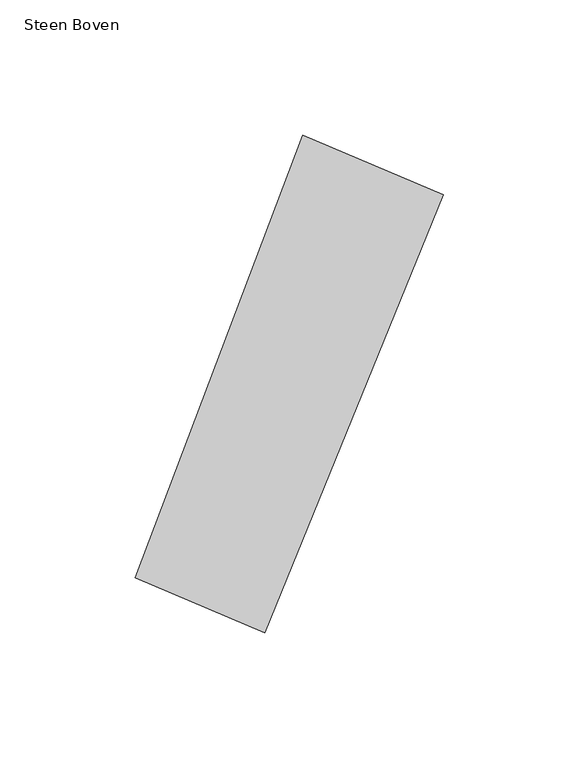
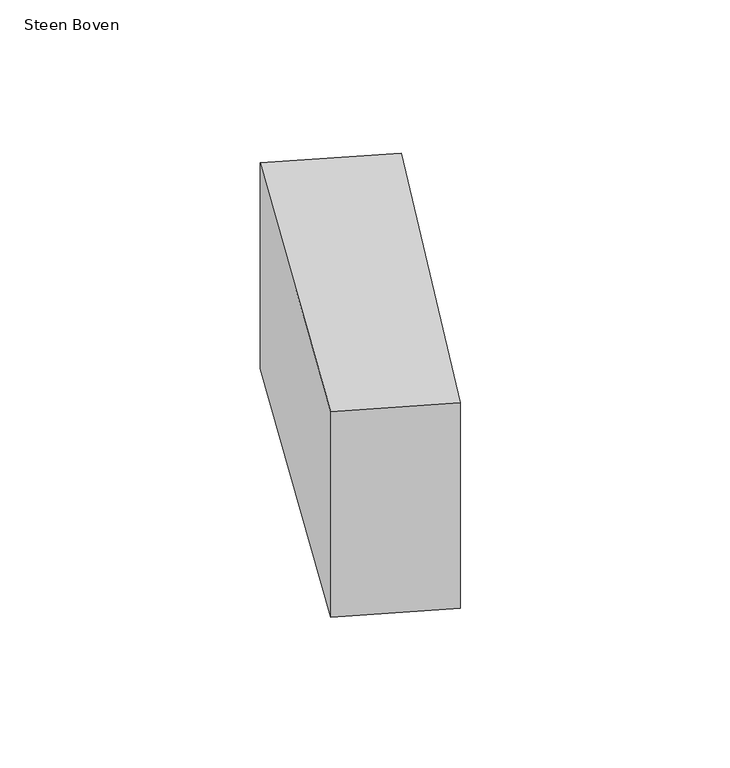
"""IFC4 building model written with IfcOpenShell, lengths in millimetres: proxy geometry, 00_GMA_steen_versie_4 : Steen Boven."""

from ifc_helpers import new_model, si_unit, origin, origin_with_axes, place, context, project, spatial, polyline, outline, extrude, source, transform, mapped, element, save


def steen_boven_43825531(model_context):
    return source(origin(), model_context, "Body", "SweptSolid", [
        extrude(outline(polyline([(135.0092648, 153.8651447), (68.783702, -8.1375562), (20.9158232, 12.1762368), (82.8466643, 176.0050232), (135.0092648, 153.8651447)])), origin_with_axes(), (0.0, 0.0, 1.0), 100.0),
    ])


if __name__ == "__main__":
    model = new_model("IFC4")
    model_context = context("Model", 3, world=origin())
    ifc_project = project(units=[si_unit("LENGTHUNIT", "METRE", prefix="MILLI")], contexts=[model_context])
    site = spatial("IfcSite", under=ifc_project)
    building = spatial("IfcBuilding", under=site)
    placement = place(None, origin())
    steen_boven_shape = steen_boven_43825531(model_context)
    element("IfcBuildingElementProxy", 1, Name="00_GMA_steen_versie_4 : Steen Boven", ObjectType="00_GMA_steen_versie_4 : Steen Boven", at=placement, inside=building, context=model_context, shape_type="MappedRepresentation", body=[
        mapped(steen_boven_shape, transform((0.0, 0.0, 0.0), x_axis=(1.0, 0.0, 0.0), y_axis=(0.0, 1.0, 0.0), z_axis=(0.0, 0.0, 1.0))),
    ])
    save(model, "model.ifc")

# Revit data of these elements
# Type "00_GMA_steen_versie_4 : Steen Boven"
#   StootVoegHalfBoven [instance default] = 5 mm
#   StootVoegHalf [instance default] = 5 mm
#   StootVoegBreedteOnder = 10 mm
#   StootVoegBreedteBoven = 10 mm
#   Steendikte = 100 mm
#   LintVoegOnderHalf = 5 mm
#   LintVoegOnder = 10 mm
#   LintVoegBovenHalf = 0 mm
#   LintVoegBoven = 0 mm
#   materiaal = none
#   MateriaalVoeg = none
#   Default Elevation = 0
